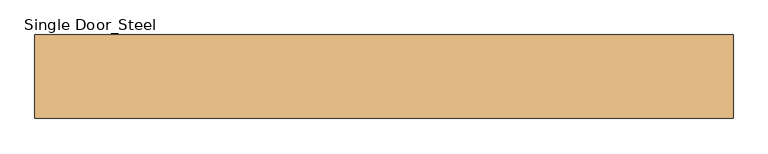
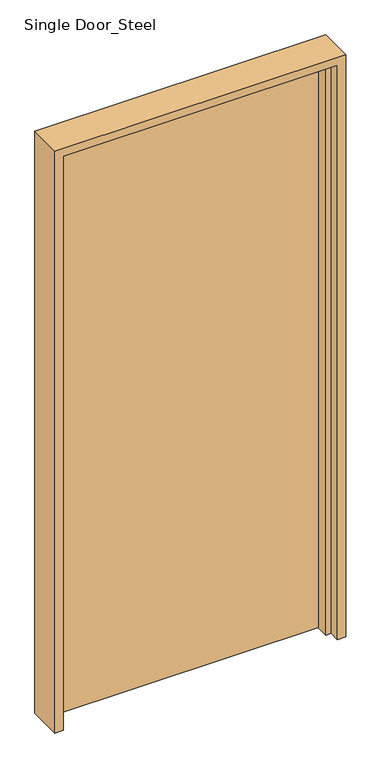
"""IFC4 building model written with IfcOpenShell, lengths in millimetres: door geometry, Single Door_Steel : H_DR_AR B12_Door_Single_W1100xH2280_No FR_SD-2."""

from ifc_helpers import new_model, si_unit, origin, origin_with_axes, place, context, project, spatial, polyline, outline, extrude, faceted_brep, source, transform, mapped, element, save


def single_door_steel_b457e09b(model_context):
    return source(origin(), model_context, "Body", "SolidModel", [
        extrude(outline(polyline([(505.0, 64.0), (505.0, 24.0), (-505.0, 24.0), (-505.0, 64.0), (505.0, 64.0)])), origin_with_axes(), (0.0, 0.0, 1.0), 2235.0),
        faceted_brep([(505.0, 64.0, 0.0), (535.0, 64.0, 0.0), (535.0, -64.0, 0.0), (505.0, -64.0, 0.0), (505.0, -24.0, 0.0), (485.0, -24.0, 0.0), (485.0, 24.0, 0.0), (505.0, 24.0, 0.0), (-505.0, 64.0, 0.0), (-505.0, 24.0, 0.0), (-485.0, 24.0, 0.0), (-485.0, -24.0, 0.0), (-505.0, -24.0, 0.0), (-505.0, -64.0, 0.0), (-535.0, -64.0, 0.0), (-535.0, 64.0, 0.0), (505.0, 64.0, 2235.0), (-505.0, 64.0, 2235.0), (-535.0, 64.0, 2265.0), (535.0, 64.0, 2265.0), (535.0, -64.0, 2265.0), (-535.0, -64.0, 2265.0), (-505.0, -64.0, 2235.0), (505.0, -64.0, 2235.0), (505.0, -24.0, 2235.0), (-505.0, -24.0, 2235.0), (-485.0, -24.0, 2215.0), (485.0, -24.0, 2215.0), (485.0, 24.0, 2215.0), (-485.0, 24.0, 2215.0), (-505.0, 24.0, 2235.0), (505.0, 24.0, 2235.0)], [[[0, 1, 2, 3, 4, 5, 6, 7]], [[8, 9, 10, 11, 12, 13, 14, 15]], [[1, 0, 16, 17, 8, 15, 18, 19]], [[2, 1, 19, 20]], [[3, 2, 20, 21, 14, 13, 22, 23]], [[4, 3, 23, 24]], [[5, 4, 24, 25, 12, 11, 26, 27]], [[6, 5, 27, 28]], [[7, 6, 28, 29, 10, 9, 30, 31]], [[0, 7, 31, 16]], [[17, 30, 9, 8]], [[21, 18, 15, 14]], [[25, 22, 13, 12]], [[29, 26, 11, 10]], [[20, 19, 18, 21]], [[24, 23, 22, 25]], [[28, 27, 26, 29]], [[16, 31, 30, 17]]]),
    ])


if __name__ == "__main__":
    model = new_model("IFC4")
    model_context = context("Model", 3, world=origin())
    ifc_project = project(units=[si_unit("LENGTHUNIT", "METRE", prefix="MILLI")], contexts=[model_context])
    site = spatial("IfcSite", under=ifc_project)
    building = spatial("IfcBuilding", under=site)
    placement = place(None, origin())
    single_door_steel_shape = single_door_steel_b457e09b(model_context)
    element("IfcDoor", 1, ObjectType="Single Door_Steel : H_DR_AR B12_Door_Single_W1100xH2280_No FR_SD-2", at=placement, inside=building, context=model_context, shape_type="MappedRepresentation", body=[
        mapped(single_door_steel_shape, transform((0.0, 0.0, 0.0), x_axis=(1.0, 0.0, 0.0), y_axis=(0.0, 1.0, 0.0), z_axis=(0.0, 0.0, 1.0))),
    ])
    save(model, "model.ifc")

# Revit data of these elements
# Type "Single Door_Steel : H_DR_AR B12_Door_Single_W1100xH2280_No FR_SD-2"
#   Type Mark = "437"
#   Analytic Construction = "<None>"
#   프레임 투영 외부. = 25 mm
#   프레임 투영 내부. = 25 mm
#   프레임 폭 = 75 mm
#   Height = 2280 mm
#   Width = 1100 mm
#   Define Thermal Properties by = 1
#   문 패널 = none
#   문 프레임 = none
#   Function = (empty or 0)
#   Wall Closure = (empty or 0)
